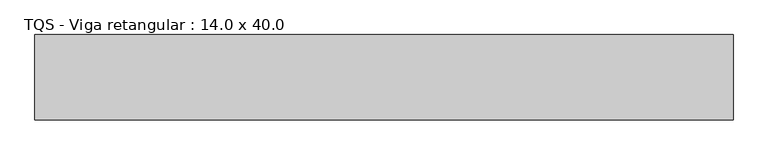
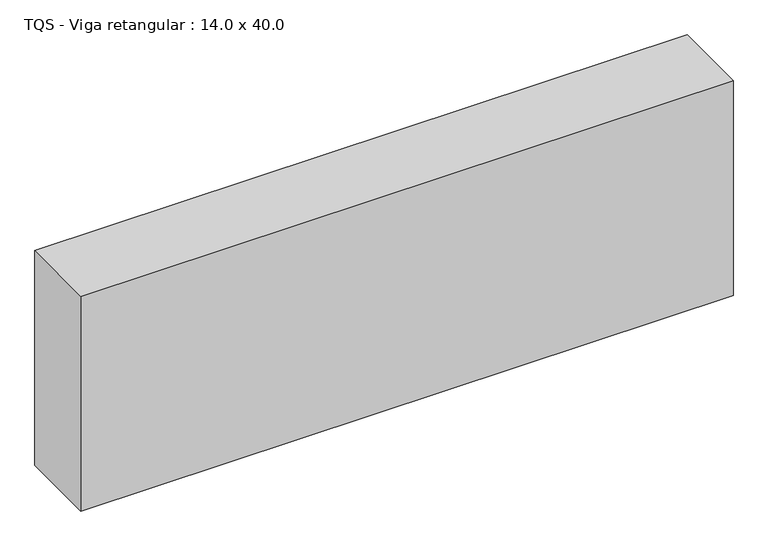
"""IFC4 building model written with IfcOpenShell, lengths in millimetres: beam geometry, TQS - Viga retangular : 14.0 x 40.0."""

import ifcopenshell
import ifcopenshell.guid

model = None  # the IFC model being written
_history = None  # IfcOwnerHistory: only IFC2X3 demands one
_inside = {}  # id of a spatial element -> (the spatial element, [elements in it])
_under = {}  # id of a project, library or spatial element -> (it, [spatial elements below it])
_declared = {}  # id of a project -> (the project, [libraries it declares])
_typed = {}  # id of a type object -> (the type object, [elements of that type])
_made_of = {}  # id of a material, layer set ... -> (it, [elements and type objects made of it])


def new_model(schema):
    """Start an empty IFC model of exactly this schema.

    Asked for "IFC4X3", IfcOpenShell would pick the latest addendum, in which some entities
    have other attributes; the version numbers below select the first issue.
    IFC2X3 requires an IfcOwnerHistory on every rooted entity: one is made here for all.
    """
    global model, _history
    if schema == "IFC4X3":
        model = ifcopenshell.file(schema_version=(4, 3, 0, 0))
    else:
        model = ifcopenshell.file(schema=schema)
    _inside.clear()
    _under.clear()
    _declared.clear()
    _typed.clear()
    _made_of.clear()
    _history = None
    if model.schema == "IFC2X3":
        org = make("IfcOrganization", Name="unknown")
        user = make(
            "IfcPersonAndOrganization",
            ThePerson=make("IfcPerson", FamilyName="unknown"),
            TheOrganization=org,
        )
        app = make(
            "IfcApplication",
            ApplicationDeveloper=org,
            Version="unknown",
            ApplicationFullName="unknown",
            ApplicationIdentifier="unknown",
        )
        _history = make(
            "IfcOwnerHistory",
            OwningUser=user,
            OwningApplication=app,
            ChangeAction="ADDED",
            CreationDate=0,
        )
    return model


def make(cls, **values):
    """One entity of the class cls with the attributes given. An attribute that is None is left unset."""
    return model.create_entity(
        cls, **{name: value for name, value in values.items() if value is not None}
    )


def rooted(cls, **values):
    """An entity with a GlobalId (a new one), such as an element, a storey or a relation."""
    return make(cls, GlobalId=ifcopenshell.guid.new(), OwnerHistory=_history, **values)


def si_unit(unit_type, name, prefix=None):
    """IfcSIUnit, for example si_unit("LENGTHUNIT", "METRE", prefix="MILLI")."""
    return make("IfcSIUnit", UnitType=unit_type, Prefix=prefix, Name=name)


def assignment(units):
    """IfcUnitAssignment: the units of a project."""
    return None if units is None else make("IfcUnitAssignment", Units=units)


def point(xyz):
    """IfcCartesianPoint."""
    return None if xyz is None else make("IfcCartesianPoint", Coordinates=xyz)


def direction(xyz):
    """IfcDirection."""
    return None if xyz is None else make("IfcDirection", DirectionRatios=xyz)


def frame(location, z_axis=None, x_axis=None):
    """IfcAxis2Placement3D, a coordinate frame: its origin and axes. An axis left out is left unset."""
    return make(
        "IfcAxis2Placement3D",
        Location=point(location),
        Axis=direction(z_axis),
        RefDirection=direction(x_axis),
    )


def origin():
    """The frame at (0, 0, 0) with its axes left unset."""
    return frame((0.0, 0.0, 0.0))


def place(relative_to, where):
    """IfcLocalPlacement: puts the frame where relative to a parent placement (None: the world)."""
    return make(
        "IfcLocalPlacement", PlacementRelTo=relative_to, RelativePlacement=where
    )


def context(
    kind, dimensions, precision=None, world=None, true_north=None, identifier=None
):
    """IfcGeometricRepresentationContext, for example the 3D "Model" context."""
    return make(
        "IfcGeometricRepresentationContext",
        ContextIdentifier=identifier,
        ContextType=kind,
        CoordinateSpaceDimension=dimensions,
        Precision=precision,
        WorldCoordinateSystem=world,
        TrueNorth=true_north,
    )


def project(units=None, contexts=None):
    """IfcProject with its units and contexts."""
    return rooted(
        "IfcProject",
        Name="project",
        RepresentationContexts=contexts,
        UnitsInContext=assignment(units),
    )


def spatial(cls, under=None, at=None, **own):
    """A site, building, storey or space (cls), placed at a placement, below another one or the project."""
    s = rooted(cls, ObjectPlacement=at, **own)
    if under is not None:
        _under.setdefault(under.id(), (under, []))[1].append(s)
    return s


def polyline(points):
    """IfcPolyline through the points."""
    return make("IfcPolyline", Points=[point(p) for p in points])


def outline(outer, holes=None, kind="AREA"):
    """IfcArbitraryClosedProfileDef: a profile drawn as a closed curve; with holes, ...WithVoids."""
    if holes is None:
        return make("IfcArbitraryClosedProfileDef", ProfileType=kind, OuterCurve=outer)
    return make(
        "IfcArbitraryProfileDefWithVoids",
        ProfileType=kind,
        OuterCurve=outer,
        InnerCurves=holes,
    )


def extrude(swept, where, along, depth):
    """IfcExtrudedAreaSolid: the profile swept, set in the frame where, extruded along a direction by depth."""
    return make(
        "IfcExtrudedAreaSolid",
        SweptArea=swept,
        Position=where,
        ExtrudedDirection=direction(along),
        Depth=depth,
    )


def shape(context_of_items, identifier, shape_type, items):
    """IfcShapeRepresentation: the items that make up one representation, for example the "Body"."""
    return make(
        "IfcShapeRepresentation",
        ContextOfItems=context_of_items,
        RepresentationIdentifier=identifier,
        RepresentationType=shape_type,
        Items=items,
    )


def source(mapping_origin, context_of_items, identifier, shape_type, items):
    """IfcRepresentationMap: a shape defined once, which mapped items show again and again."""
    return make(
        "IfcRepresentationMap",
        MappingOrigin=mapping_origin,
        MappedRepresentation=shape(context_of_items, identifier, shape_type, items),
    )


def transform(
    local_origin,
    x_axis=None,
    y_axis=None,
    z_axis=None,
    scale=None,
    scale2=None,
    scale3=None,
    uniform=True,
):
    """IfcCartesianTransformationOperator3D, or its non-uniform kind. x_axis, y_axis, z_axis: its Axis1, 2, 3."""
    if uniform:
        return make(
            "IfcCartesianTransformationOperator3D",
            Axis1=direction(x_axis),
            Axis2=direction(y_axis),
            LocalOrigin=point(local_origin),
            Scale=scale,
            Axis3=direction(z_axis),
        )
    return make(
        "IfcCartesianTransformationOperator3DnonUniform",
        Axis1=direction(x_axis),
        Axis2=direction(y_axis),
        LocalOrigin=point(local_origin),
        Scale=scale,
        Axis3=direction(z_axis),
        Scale2=scale2,
        Scale3=scale3,
    )


def mapped(mapping_source, mapping_target):
    """IfcMappedItem: shows the shape of a source again, moved by a transform."""
    return make(
        "IfcMappedItem", MappingSource=mapping_source, MappingTarget=mapping_target
    )


def made_of(thing, what):
    """Note that an element or type object is made of a material, layer set ...; save() writes the relation."""
    if what is not None:
        _made_of.setdefault(what.id(), (what, []))[1].append(thing)
    return thing


def element(
    cls,
    number,
    at=None,
    inside=None,
    cuts=None,
    type_object=None,
    material=None,
    context=None,
    identifier="Body",
    shape_type=None,
    held_by="IfcProductDefinitionShape",
    body=None,
    shapes=None,
    **own,
):
    """One element of the class cls, such as IfcWall. Its Tag is "e" and its number.

    at: its placement. inside: the storey or other place that contains it. cuts: it is an
    opening in that element (IfcRelVoidsElement). A single representation is given by context,
    identifier, shape_type and body (its items); several are given by shapes. held_by: the class
    of the entity that holds the representations. save() writes the other relations.
    """
    e = rooted(cls, Tag="e%d" % number, ObjectPlacement=at, **own)
    if body is not None:
        shapes = [shape(context, identifier, shape_type, body)]
    if shapes is not None:
        e.Representation = make(held_by, Representations=shapes)
    if inside is not None:
        _inside.setdefault(inside.id(), (inside, []))[1].append(e)
    if cuts is not None:
        rooted(
            "IfcRelVoidsElement", RelatingBuildingElement=cuts, RelatedOpeningElement=e
        )
    if type_object is not None:
        _typed.setdefault(type_object.id(), (type_object, []))[1].append(e)
    return made_of(e, material)


def aggregate(whole, parts):
    """IfcRelAggregates: a whole, such as a stair, and the parts it consists of."""
    return rooted("IfcRelAggregates", RelatingObject=whole, RelatedObjects=parts)


def save(model, path):
    """Write the relations noted so far, then the file.

    IfcRelAggregates (storeys below a building ...), IfcRelContainedInSpatialStructure (elements
    in a storey), IfcRelDefinesByType, IfcRelAssociatesMaterial and IfcRelDeclares: one each for
    every whole, place, type object, material and project.
    """
    for whole, parts in _under.values():
        aggregate(whole, parts)
    for where, things in _inside.values():
        rooted(
            "IfcRelContainedInSpatialStructure",
            RelatedElements=things,
            RelatingStructure=where,
        )
    for kind, things in _typed.values():
        rooted("IfcRelDefinesByType", RelatedObjects=things, RelatingType=kind)
    for what, things in _made_of.values():
        rooted("IfcRelAssociatesMaterial", RelatedObjects=things, RelatingMaterial=what)
    for by, libraries in _declared.values():
        rooted("IfcRelDeclares", RelatingContext=by, RelatedDefinitions=libraries)
    model.write(path)


def tqs_viga_retangular_14_0_x_40_0_8fae01fb(model_context):
    return source(origin(), model_context, "Body", "SweptSolid", [
        extrude(outline(polyline([(573.9, 70.0), (573.9, -70.0), (-573.9, -70.0), (-573.9, 70.0), (573.9, 70.0)])), frame((0.0, 0.0, -200.0), z_axis=(0.0, 0.0, 1.0), x_axis=(1.0, 0.0, 0.0)), (0.0, 0.0, 1.0), 400.0),
    ])


if __name__ == "__main__":
    model = new_model("IFC4")
    model_context = context("Model", 3, world=origin())
    ifc_project = project(units=[si_unit("LENGTHUNIT", "METRE", prefix="MILLI")], contexts=[model_context])
    site = spatial("IfcSite", under=ifc_project)
    building = spatial("IfcBuilding", under=site)
    placement = place(None, origin())
    tqs_viga_retangular_14_0_x_40_0_shape = tqs_viga_retangular_14_0_x_40_0_8fae01fb(model_context)
    element("IfcBeam", 1, ObjectType="TQS - Viga retangular : 14.0 x 40.0", at=placement, inside=building, context=model_context, shape_type="MappedRepresentation", body=[
        mapped(tqs_viga_retangular_14_0_x_40_0_shape, transform((0.0, 0.0, 0.0), x_axis=(1.0, 0.0, 0.0), y_axis=(0.0, 1.0, 0.0), z_axis=(0.0, 0.0, 1.0))),
    ])
    save(model, "model.ifc")

# Revit data of these elements
# Type "TQS - Viga retangular : 14.0 x 40.0"
#   Length [instance default] = 1.524 m
#   b = 0.14 m
#   h = 0.40 m
#   Structural Material [instance default] = none
#   Assembly Code = ""
